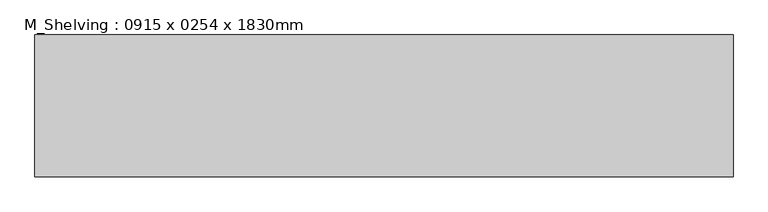
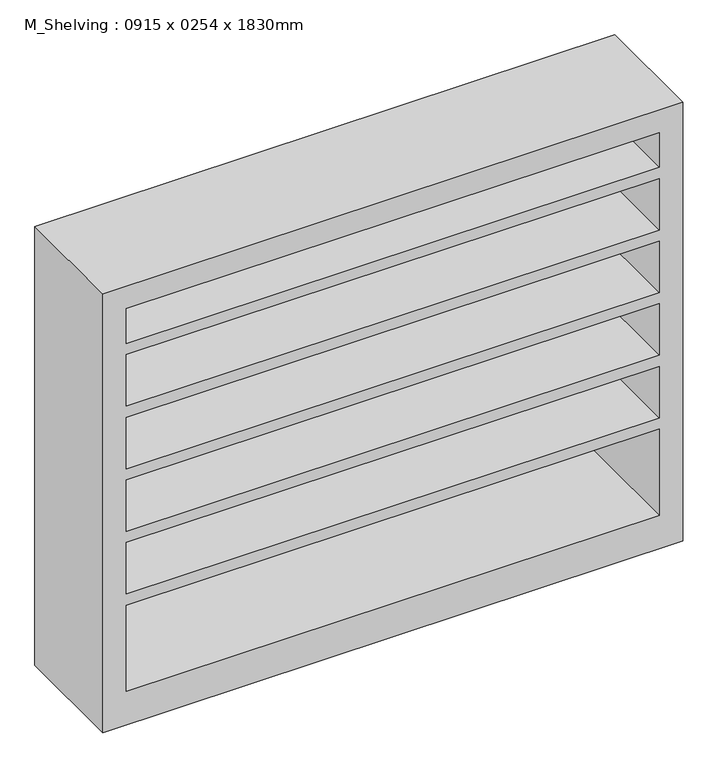
"""IFC4 building model written with IfcOpenShell, lengths in millimetres: furniture geometry, M_Shelving : 0915 x 0254 x 1830mm."""

from ifc_helpers import new_model, si_unit, frame, origin, place, context, project, spatial, polyline, outline, extrude, source, transform, mapped, element, save


def m_shelving_0915_x_0254_x_1830mm_07cf747d(model_context):
    return source(origin(), model_context, "Body", "SweptSolid", [
        extrude(outline(polyline([(0.0, 625.0), (1000.0, 625.0), (1000.0, -625.0), (0.0, -625.0), (0.0, 625.0)]), holes=[polyline([(949.2, 574.2), (869.8428571, 574.2), (869.8428571, -574.2), (949.2, -574.2), (949.2, 574.2)]), polyline([(76.2, 574.2), (76.2, -574.2), (273.0142857, -574.2), (273.0142857, 574.2), (76.2, 574.2)]), polyline([(584.1285714, -574.2), (701.5857143, -574.2), (701.5857143, 574.2), (584.1285714, 574.2), (584.1285714, -574.2)]), polyline([(844.4428571, 574.2), (726.9857143, 574.2), (726.9857143, -574.2), (844.4428571, -574.2), (844.4428571, 574.2)]), polyline([(558.7285714, 574.2), (441.2714286, 574.2), (441.2714286, -574.2), (558.7285714, -574.2), (558.7285714, 574.2)]), polyline([(415.8714286, 574.2), (298.4142857, 574.2), (298.4142857, -574.2), (415.8714286, -574.2), (415.8714286, 574.2)])]), frame((0.0, -431.8, 0.0), z_axis=(0.0, 1.0, 0.0), x_axis=(0.0, 0.0, 1.0)), (0.0, 0.0, 1.0), 254.0),
    ])


if __name__ == "__main__":
    model = new_model("IFC4")
    model_context = context("Model", 3, world=origin())
    ifc_project = project(units=[si_unit("LENGTHUNIT", "METRE", prefix="MILLI")], contexts=[model_context])
    site = spatial("IfcSite", under=ifc_project)
    building = spatial("IfcBuilding", under=site)
    placement = place(None, origin())
    m_shelving_0915_x_0254_x_1830mm_shape = m_shelving_0915_x_0254_x_1830mm_07cf747d(model_context)
    element("IfcFurniture", 1, ObjectType="M_Shelving : 0915 x 0254 x 1830mm", at=placement, inside=building, context=model_context, shape_type="MappedRepresentation", body=[
        mapped(m_shelving_0915_x_0254_x_1830mm_shape, transform((0.0, 0.0, 0.0), x_axis=(1.0, 0.0, 0.0), y_axis=(0.0, 1.0, 0.0), z_axis=(0.0, 0.0, 1.0))),
    ])
    save(model, "model.ifc")

# Revit data of these elements
# Type "M_Shelving : 0915 x 0254 x 1830mm"
#   Depth = 0.254 m
#   Height = 1 m
#   Width = 1.25 m
#   Material = Birch
# Element 1 (IfcFurniture, "M_Shelving : 0915 x 0254 x 1830mm")
#   Materials on its faces: "Birch"
# Materials
#   "Birch": class "Wood", colour RGB 224 178 126, transparency 0, Description = "Betula Alleghaniensis", Cost = 0
